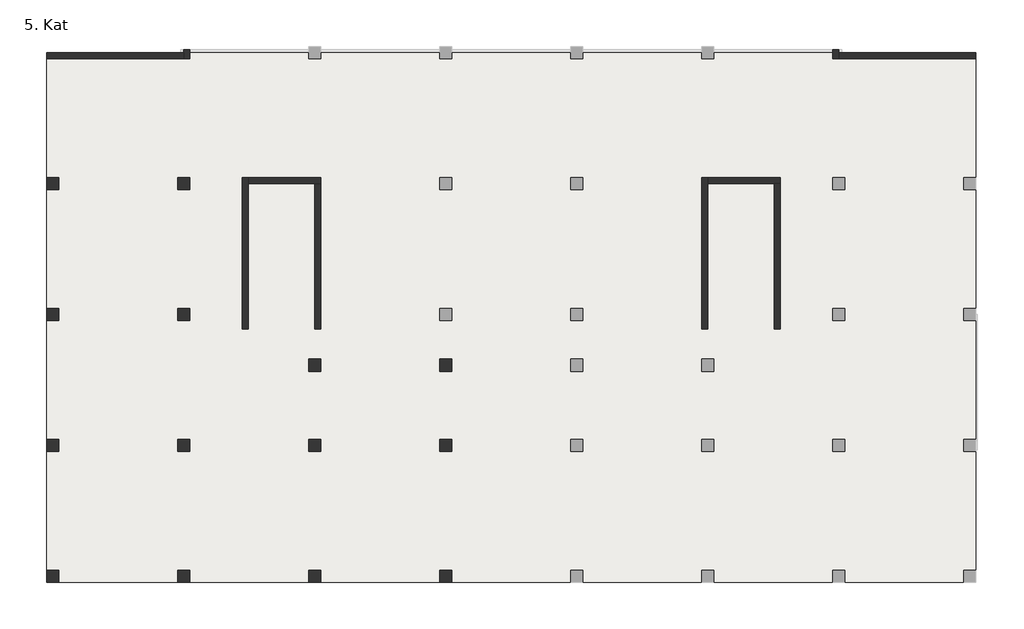
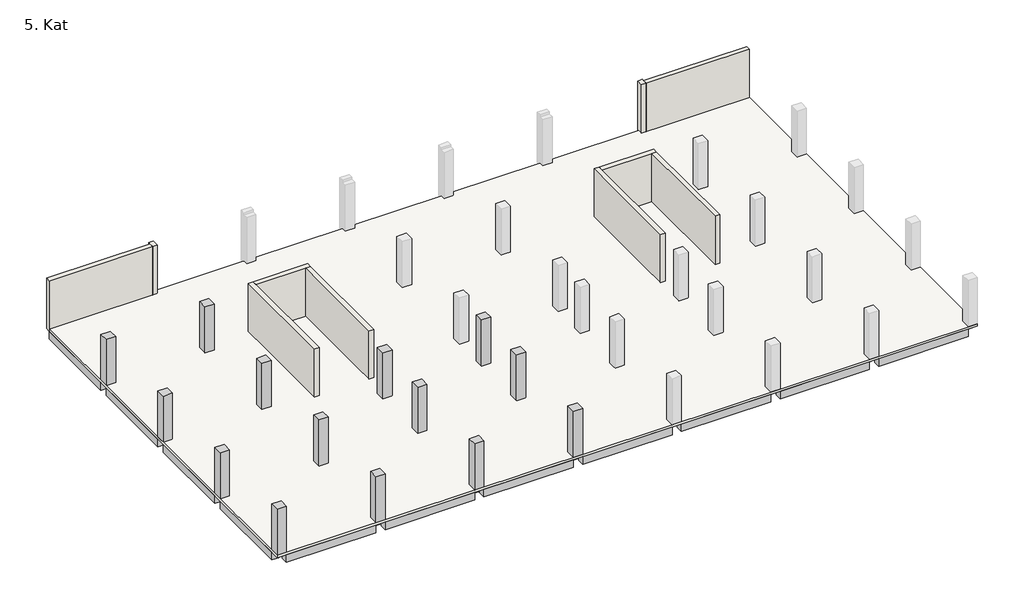
# One storey, part 1 of 2: 41 beams, 14 columns, 10 walls, 1 slab.
"""IFC4 building model written with IfcOpenShell, lengths in millimetres."""

from ifc_helpers import new_model, si_unit, frame, origin, place, context, project, spatial, polyline, outline, extrude, faceted_brep, element, save

model = new_model("IFC4")

# Units and contexts
model_context = context("Model", 3, world=origin())
ifc_project = project(units=[si_unit("LENGTHUNIT", "METRE", prefix="MILLI")], contexts=[model_context])

# Site, building, storey
site = spatial("IfcSite", under=ifc_project)
building = spatial("IfcBuilding", under=site)
storey = spatial("IfcBuildingStorey", under=building, Name="5. Kat", Elevation=26500.0)

# Beams
placement = place(None, origin())
element("IfcBeam", 1, ObjectType="M_Concrete-Rectangular Beam : 60x70cm kiriş", at=placement, inside=storey, context=model_context, shape_type="SweptSolid", body=[
    extrude(outline(polyline([(-400.0003889, 8099.9999582), (199.9996111, 8099.9999582), (199.9996111, 399.9999408), (-400.0003889, 399.9999408), (-400.0003889, 8099.9999582)])), frame((0.0, 0.0, 25800.0), z_axis=(0.0, 0.0, 1.0), x_axis=(1.0, 0.0, 0.0)), (0.0, 0.0, 1.0), 700.0),
])
element("IfcBeam", 2, ObjectType="M_Concrete-Rectangular Beam : 60x70cm kiriş", at=placement, inside=storey, context=model_context, shape_type="SweptSolid", body=[
    extrude(outline(polyline([(-400.0003589, 16599.9999423), (199.9996411, 16599.9999423), (199.9996411, 8899.9999251), (-400.0003589, 8899.9999251), (-400.0003589, 16599.9999423)])), frame((0.0, 0.0, 25800.0), z_axis=(0.0, 0.0, 1.0), x_axis=(1.0, 0.0, 0.0)), (0.0, 0.0, 1.0), 700.0),
])
element("IfcBeam", 3, ObjectType="M_Concrete-Rectangular Beam : 60x70cm kiriş", at=placement, inside=storey, context=model_context, shape_type="Brep", body=[
    faceted_brep([(199.9994072, 25099.999926, 26500.0), (-400.0005928, 25099.999926, 26500.0), (-400.0005928, 17399.9999423, 26500.0), (199.9994072, 17399.9999423, 26500.0), (199.9994072, 23399.9999249, 26500.0), (199.9994072, 23899.9999249, 26500.0), (199.9994072, 25099.999926, 25800.0), (199.9994072, 17399.9999423, 25800.0), (199.9994072, 23399.9999249, 25800.0), (199.9994072, 23899.9999249, 25800.0), (-400.0005928, 25099.999926, 25800.0), (-400.0005928, 17399.9999423, 25800.0)], [[[0, 1, 2, 3, 4, 5]], [[6, 0, 5, 4, 3, 7, 8, 9]], [[10, 6, 9, 8, 7, 11]], [[1, 10, 11, 2]], [[2, 11, 7, 3]], [[1, 0, 6, 10]]]),
])
element("IfcBeam", 4, ObjectType="M_Concrete-Rectangular Beam : 60x70cm kiriş", at=placement, inside=storey, context=model_context, shape_type="SweptSolid", body=[
    extrude(outline(polyline([(199.9994681, 25899.9999188), (-400.0005319, 25899.9999188), (-400.0005319, 33600.0004302), (199.9994681, 33600.0004302), (199.9994681, 25899.9999188)])), frame((0.0, 0.0, 25800.0), z_axis=(0.0, 0.0, 1.0), x_axis=(1.0, 0.0, 0.0)), (0.0, 0.0, 1.0), 700.0),
])
element("IfcBeam", 5, ObjectType="M_Concrete-Rectangular Beam : 60x70cm kiriş", at=placement, inside=storey, context=model_context, shape_type="SweptSolid", body=[
    extrude(outline(polyline([(8099.9996095, 199.9995192), (8099.9996095, -400.0004808), (399.9996111, -400.0004808), (399.9996111, 199.9995192), (8099.9996095, 199.9995192)])), frame((0.0, 0.0, 25800.0), z_axis=(0.0, 0.0, 1.0), x_axis=(1.0, 0.0, 0.0)), (0.0, 0.0, 1.0), 700.0),
])
element("IfcBeam", 6, ObjectType="M_Concrete-Rectangular Beam : 60x70cm kiriş", at=placement, inside=storey, context=model_context, shape_type="SweptSolid", body=[
    extrude(outline(polyline([(16599.9996095, 199.9999577), (16599.9996095, -400.0000423), (8899.9996095, -400.0000423), (8899.9996095, 199.9999577), (16599.9996095, 199.9999577)])), frame((0.0, 0.0, 25800.0), z_axis=(0.0, 0.0, 1.0), x_axis=(1.0, 0.0, 0.0)), (0.0, 0.0, 1.0), 700.0),
])
element("IfcBeam", 7, ObjectType="M_Concrete-Rectangular Beam : 60x70cm kiriş", at=placement, inside=storey, context=model_context, shape_type="SweptSolid", body=[
    extrude(outline(polyline([(25099.9996096, 200.0003837), (25099.9996096, -399.9996163), (17399.9993907, -399.9996163), (17399.9993907, 200.0003837), (25099.9996096, 200.0003837)])), frame((0.0, 0.0, 25800.0), z_axis=(0.0, 0.0, 1.0), x_axis=(1.0, 0.0, 0.0)), (0.0, 0.0, 1.0), 700.0),
])
element("IfcBeam", 8, ObjectType="M_Concrete-Rectangular Beam : 60x70cm kiriş", at=placement, inside=storey, context=model_context, shape_type="SweptSolid", body=[
    extrude(outline(polyline([(8299.9996095, 8100.0003637), (8899.9996095, 8100.0003637), (8899.9996095, 399.9999384), (8299.9996095, 399.9999384), (8299.9996095, 8100.0003637)])), frame((0.0, 0.0, 25800.0), z_axis=(0.0, 0.0, 1.0), x_axis=(1.0, 0.0, 0.0)), (0.0, 0.0, 1.0), 700.0),
])
element("IfcBeam", 9, ObjectType="M_Concrete-Rectangular Beam : 60x70cm kiriş", at=placement, inside=storey, context=model_context, shape_type="Brep", body=[
    faceted_brep([(8899.9996095, 16599.9999418, 26500.0), (8299.9996095, 16599.9999418, 26500.0), (8299.9996095, 8900.0003637, 26500.0), (8899.9996095, 8900.0003637, 26500.0), (8899.9996095, 13300.0003638, 26500.0), (8899.9996095, 13700.0003638, 26500.0), (8899.9996095, 16599.9999418, 25800.0), (8899.9996095, 8900.0003637, 25800.0), (8899.9996095, 13300.0003638, 25800.0), (8899.9996095, 13700.0003638, 25800.0), (8299.9996095, 16599.9999418, 25800.0), (8299.9996095, 8900.0003637, 25800.0)], [[[0, 1, 2, 3, 4, 5]], [[6, 0, 5, 4, 3, 7, 8, 9]], [[10, 6, 9, 8, 7, 11]], [[1, 10, 11, 2]], [[2, 11, 7, 3]], [[1, 0, 6, 10]]]),
])
element("IfcBeam", 10, ObjectType="M_Concrete-Rectangular Beam : 60x70cm kiriş", at=placement, inside=storey, context=model_context, shape_type="Brep", body=[
    faceted_brep([(8899.9996735, 25100.0003646, 26500.0), (8299.9996735, 25100.0003646, 26500.0), (8299.9996735, 23899.9999249, 26500.0), (8299.9996735, 23399.9999249, 26500.0), (8299.9996735, 18550.0006424, 26500.0), (8299.9996735, 18150.0006424, 26500.0), (8299.9996735, 17400.0009197, 26500.0), (8899.9996735, 17400.0009197, 26500.0), (8899.9996735, 25100.0003646, 25800.0), (8899.9996735, 17400.0009197, 25800.0), (8299.9996735, 25100.0003646, 25800.0), (8299.9996735, 17400.0009197, 25800.0), (8299.9996735, 18150.0006424, 25800.0), (8299.9996735, 18550.0006424, 25800.0), (8299.9996735, 23399.9999249, 25800.0), (8299.9996735, 23899.9999249, 25800.0)], [[[0, 1, 2, 3, 4, 5, 6, 7]], [[8, 0, 7, 9]], [[10, 8, 9, 11, 12, 13, 14, 15]], [[1, 10, 15, 14, 13, 12, 11, 6, 5, 4, 3, 2]], [[1, 0, 8, 10]], [[7, 6, 11, 9]]]),
])
element("IfcBeam", 11, ObjectType="M_Concrete-Rectangular Beam : 60x70cm kiriş", at=placement, inside=storey, context=model_context, shape_type="Brep", body=[
    faceted_brep([(8299.9993907, 25899.9999188, 26500.0), (8899.9993907, 25899.9999188, 26500.0), (8899.9993907, 33600.0004302, 26500.0), (8499.9995273, 33600.0004302, 26500.0), (8299.9993907, 33600.0004302, 26500.0), (8899.9993907, 25899.9999188, 25800.0), (8899.9993907, 33600.0004302, 25800.0), (8299.9993907, 25899.9999188, 25800.0), (8299.9993907, 33600.0004302, 25800.0)], [[[0, 1, 2, 3, 4]], [[1, 5, 6, 2]], [[5, 7, 8, 6]], [[7, 0, 4, 8]], [[5, 1, 0, 7]], [[8, 4, 3, 2, 6]]]),
])
element("IfcBeam", 12, ObjectType="M_Concrete-Rectangular Beam : 60x70cm kiriş", at=placement, inside=storey, context=model_context, shape_type="SweptSolid", body=[
    extrude(outline(polyline([(8099.9997323, 25899.999992), (8099.9997323, 25299.999992), (399.9997323, 25299.999992), (399.9997323, 25899.999992), (8099.9997323, 25899.999992)])), frame((0.0, 0.0, 25800.0), z_axis=(0.0, 0.0, 1.0), x_axis=(1.0, 0.0, 0.0)), (0.0, 0.0, 1.0), 700.0),
])
element("IfcBeam", 13, ObjectType="M_Concrete-Rectangular Beam : 50x70cm kiriş", at=placement, inside=storey, context=model_context, shape_type="SweptSolid", body=[
    extrude(outline(polyline([(199.9994072, 23399.9999249), (199.9994072, 23899.9999249), (8299.9996735, 23899.9999249), (8299.9996735, 23399.9999249), (199.9994072, 23399.9999249)])), frame((0.0, 0.0, 25800.0), z_axis=(0.0, 0.0, 1.0), x_axis=(1.0, 0.0, 0.0)), (0.0, 0.0, 1.0), 700.0),
])
element("IfcBeam", 14, ObjectType="M_Concrete-Rectangular Beam : 60x70cm kiriş", at=placement, inside=storey, context=model_context, shape_type="SweptSolid", body=[
    extrude(outline(polyline([(8099.9997451, 8800.0009197), (8099.9997451, 8200.0009197), (399.9996411, 8200.0009197), (399.9996411, 8800.0009197), (8099.9997451, 8800.0009197)])), frame((0.0, 0.0, 25800.0), z_axis=(0.0, 0.0, 1.0), x_axis=(1.0, 0.0, 0.0)), (0.0, 0.0, 1.0), 700.0),
])
element("IfcBeam", 15, ObjectType="M_Concrete-Rectangular Beam : 60x70cm kiriş", at=placement, inside=storey, context=model_context, shape_type="SweptSolid", body=[
    extrude(outline(polyline([(8099.9993907, 17400.0003638), (8099.9993907, 16800.0003638), (400.0000836, 16800.0003638), (400.0000836, 17400.0003638), (8099.9993907, 17400.0003638)])), frame((0.0, 0.0, 25800.0), z_axis=(0.0, 0.0, 1.0), x_axis=(1.0, 0.0, 0.0)), (0.0, 0.0, 1.0), 700.0),
])
element("IfcBeam", 16, ObjectType="M_Concrete-Rectangular Beam : 40x70cm kiriş 2", at=placement, inside=storey, context=model_context, shape_type="SweptSolid", body=[
    extrude(outline(polyline([(204.0222331, 18150.0006424), (204.0222331, 18550.0006424), (8299.9996735, 18550.0006424), (8299.9996735, 18150.0006424), (204.0222331, 18150.0006424)])), frame((0.0, 0.0, 25800.0), z_axis=(0.0, 0.0, 1.0), x_axis=(1.0, 0.0, 0.0)), (0.0, 0.0, 1.0), 700.0),
])
element("IfcBeam", 17, ObjectType="M_Concrete-Rectangular Beam : 60x70cm kiriş", at=placement, inside=storey, context=model_context, shape_type="Brep", body=[
    faceted_brep([(8899.9993907, 25899.9999925, 26500.0), (8899.9993907, 25299.9999925, 26500.0), (12300.0064017, 25299.9999925, 26500.0), (12300.0064017, 25500.0003816, 26500.0), (12300.0064017, 25899.9999925, 26500.0), (8899.9993907, 25299.9999925, 25800.0), (12300.0064017, 25299.9999925, 25800.0), (8899.9993907, 25899.9999925, 25800.0), (12300.0064017, 25899.9999925, 25800.0)], [[[0, 1, 2, 3, 4]], [[1, 5, 6, 2]], [[5, 7, 8, 6]], [[7, 0, 4, 8]], [[0, 7, 5, 1]], [[4, 3, 2, 6, 8]]]),
])
element("IfcBeam", 18, ObjectType="M_Concrete-Rectangular Beam : 60x70cm kiriş", at=placement, inside=storey, context=model_context, shape_type="Brep", body=[
    faceted_brep([(8899.9996735, 17400.0003643, 26500.0), (8899.9993907, 16800.0003643, 26500.0), (12300.0064017, 16800.0003643, 26500.0), (12300.0064017, 17400.0003643, 26500.0), (8899.9993907, 16800.0003643, 25800.0), (12300.0064017, 16800.0003643, 25800.0), (8899.9996735, 17400.0003643, 25800.0), (12300.0064017, 17400.0003643, 25800.0)], [[[0, 1, 2, 3]], [[1, 4, 5, 2]], [[4, 6, 7, 5]], [[6, 0, 3, 7]], [[0, 6, 4, 1]], [[3, 2, 5, 7]]]),
])
element("IfcBeam", 19, ObjectType="M_Concrete-Rectangular Beam : 40x70cm kiriş 2", at=placement, inside=storey, context=model_context, shape_type="Brep", body=[
    faceted_brep([(12700.0064017, 17400.0003638, 26500.0), (12700.0064017, 17000.0003638, 26500.0), (14600.0010318, 17000.0003638, 26500.0), (14900.0010318, 17000.0003638, 26500.0), (16999.9995362, 17000.0003638, 26500.0), (16999.9995362, 17400.0003638, 26500.0), (12700.0064017, 17000.0003638, 25800.0), (14600.0010318, 17000.0003638, 25800.0), (14900.0010318, 17000.0003638, 25800.0), (16999.9995362, 17000.0003638, 25800.0), (12700.0064017, 17400.0003638, 25800.0), (16999.9995362, 17400.0003638, 25800.0)], [[[0, 1, 2, 3, 4, 5]], [[1, 6, 7, 8, 9, 4, 3, 2]], [[6, 10, 11, 9, 8, 7]], [[10, 0, 5, 11]], [[1, 0, 10, 6]], [[5, 4, 9, 11]]]),
])
element("IfcBeam", 20, ObjectType="M_Concrete-Rectangular Beam : 40x70cm kiriş 2", at=placement, inside=storey, context=model_context, shape_type="Brep", body=[
    faceted_brep([(16599.9993867, 13300.0003638, 26500.0), (16599.9993867, 13700.0003638, 26500.0), (14900.0010318, 13700.0003638, 26500.0), (14600.0010318, 13700.0003638, 26500.0), (12700.0064017, 13700.0003638, 26500.0), (12300.0064017, 13700.0003638, 26500.0), (8899.9996095, 13700.0003638, 26500.0), (8899.9996095, 13300.0003638, 26500.0), (12300.0064017, 13300.0003638, 26500.0), (12700.0064017, 13300.0003638, 26500.0), (16599.9993867, 13700.0003638, 25800.0), (14900.0010318, 13700.0003638, 25800.0), (14600.0010318, 13700.0003638, 25800.0), (12700.0064017, 13700.0003638, 25800.0), (12300.0064017, 13700.0003638, 25800.0), (8899.9996095, 13700.0003638, 25800.0), (16599.9993867, 13300.0003638, 25800.0), (12700.0064017, 13300.0003638, 25800.0), (12300.0064017, 13300.0003638, 25800.0), (8899.9996095, 13300.0003638, 25800.0)], [[[0, 1, 2, 3, 4, 5, 6, 7, 8, 9]], [[1, 10, 11, 12, 13, 14, 15, 6, 5, 4, 3, 2]], [[10, 16, 17, 18, 19, 15, 14, 13, 12, 11]], [[16, 0, 9, 8, 7, 19, 18, 17]], [[7, 6, 15, 19]], [[0, 16, 10, 1]]]),
])
element("IfcBeam", 21, ObjectType="M_Concrete-Rectangular Beam : 40x70cm kiriş 2", at=placement, inside=storey, context=model_context, shape_type="SweptSolid", body=[
    extrude(outline(polyline([(12300.0064017, 16037.3003638), (12700.0064017, 16037.3003638), (12700.0064017, 13700.0003638), (12300.0064017, 13700.0003638), (12300.0064017, 16037.3003638)])), frame((0.0, 0.0, 25800.0), z_axis=(0.0, 0.0, 1.0), x_axis=(1.0, 0.0, 0.0)), (0.0, 0.0, 1.0), 700.0),
])
element("IfcBeam", 22, ObjectType="M_Concrete-Rectangular Beam : 40x70cm kiriş 2", at=placement, inside=storey, context=model_context, shape_type="SweptSolid", body=[
    extrude(outline(polyline([(17399.9995362, 14099.9451047), (16999.9995362, 14099.9451047), (16999.9995362, 16037.3003638), (17399.9995362, 16037.3003638), (17399.9995362, 14099.9451047)])), frame((0.0, 0.0, 25800.0), z_axis=(0.0, 0.0, 1.0), x_axis=(1.0, 0.0, 0.0)), (0.0, 0.0, 1.0), 700.0),
])
element("IfcBeam", 23, ObjectType="M_Concrete-Rectangular Beam : 30x70cm kiriş 3", at=placement, inside=storey, context=model_context, shape_type="Brep", body=[
    faceted_brep([(12700.0064017, 16350.0003638, 26500.0), (12700.0064017, 16050.0003638, 26500.0), (14600.0010318, 16050.0003638, 26500.0), (14900.0010318, 16050.0003638, 26500.0), (16999.9995362, 16050.0003638, 26500.0), (16999.9995362, 16350.0003638, 26500.0), (14900.0010318, 16350.0003638, 26500.0), (14600.0010318, 16350.0003638, 26500.0), (12700.0064017, 16350.0003638, 25800.0), (16999.9995362, 16350.0003638, 25800.0), (14900.0010318, 16350.0003638, 25800.0), (14600.0010318, 16350.0003638, 25800.0), (12700.0064017, 16050.0003638, 25800.0), (16999.9995362, 16050.0003638, 25800.0), (14900.0010318, 16050.0003638, 25800.0), (14600.0010318, 16050.0003638, 25800.0)], [[[0, 1, 2, 3, 4, 5, 6, 7]], [[8, 0, 7, 6, 5, 9, 10, 11]], [[12, 8, 11, 10, 9, 13, 14, 15]], [[1, 12, 15, 14, 13, 4, 3, 2]], [[0, 8, 12, 1]], [[5, 4, 13, 9]]]),
])
element("IfcBeam", 24, ObjectType="M_Concrete-Rectangular Beam : 30x70cm kiriş 3", at=placement, inside=storey, context=model_context, shape_type="SweptSolid", body=[
    extrude(outline(polyline([(14900.0010318, 13700.0003638), (14600.0010318, 13700.0003638), (14600.0010318, 16050.0003638), (14900.0010318, 16050.0003638), (14900.0010318, 13700.0003638)])), frame((0.0, 0.0, 25800.0), z_axis=(0.0, 0.0, 1.0), x_axis=(1.0, 0.0, 0.0)), (0.0, 0.0, 1.0), 700.0),
    extrude(outline(polyline([(14600.0010318, 17000.0003638), (14900.0010318, 17000.0003638), (14900.0010318, 16350.0003638), (14600.0010318, 16350.0003638), (14600.0010318, 17000.0003638)])), frame((0.0, 0.0, 25800.0), z_axis=(0.0, 0.0, 1.0), x_axis=(1.0, 0.0, 0.0)), (0.0, 0.0, 1.0), 700.0),
])
element("IfcBeam", 25, ObjectType="M_Concrete-Rectangular Beam : 60x70cm kiriş", at=placement, inside=storey, context=model_context, shape_type="Brep", body=[
    faceted_brep([(16599.9993907, 8200.0009197, 26500.0), (16599.9993907, 8800.0009197, 26500.0), (12700.0064017, 8800.0009197, 26500.0), (12300.0064017, 8800.0009197, 26500.0), (8899.9993907, 8800.0009197, 26500.0), (8899.9993907, 8200.0009197, 26500.0), (16599.9993907, 8200.0009197, 25800.0), (8899.9993907, 8200.0009197, 25800.0), (16599.9993907, 8800.0009197, 25800.0), (8899.9993907, 8800.0009197, 25800.0), (12300.0064017, 8800.0009197, 25800.0), (12700.0064017, 8800.0009197, 25800.0)], [[[0, 1, 2, 3, 4, 5]], [[6, 0, 5, 7]], [[8, 6, 7, 9, 10, 11]], [[1, 8, 11, 10, 9, 4, 3, 2]], [[4, 9, 7, 5]], [[1, 0, 6, 8]]]),
])
element("IfcBeam", 26, ObjectType="M_Concrete-Rectangular Beam : 60x70cm kiriş", at=placement, inside=storey, context=model_context, shape_type="SweptSolid", body=[
    extrude(outline(polyline([(17399.9997293, 8900.0009197), (16799.9997293, 8900.0009197), (16799.9997293, 13299.9451047), (17399.9997293, 13299.9451047), (17399.9997293, 8900.0009197)])), frame((0.0, 0.0, 25800.0), z_axis=(0.0, 0.0, 1.0), x_axis=(1.0, 0.0, 0.0)), (0.0, 0.0, 1.0), 700.0),
])
element("IfcBeam", 27, ObjectType="M_Concrete-Rectangular Beam : 60x70cm kiriş", at=placement, inside=storey, context=model_context, shape_type="SweptSolid", body=[
    extrude(outline(polyline([(17399.9997451, 400.0009197), (16799.9997451, 400.0009197), (16799.9997451, 8099.9999409), (17399.9997451, 8099.9999409), (17399.9997451, 400.0009197)])), frame((0.0, 0.0, 25800.0), z_axis=(0.0, 0.0, 1.0), x_axis=(1.0, 0.0, 0.0)), (0.0, 0.0, 1.0), 700.0),
])
element("IfcBeam", 28, ObjectType="M_Concrete-Rectangular Beam : 40x70cm kiriş 2", at=placement, inside=storey, context=model_context, shape_type="SweptSolid", body=[
    extrude(outline(polyline([(12300.0064017, 13300.0003638), (12700.0064017, 13300.0003638), (12700.0064017, 8800.0009197), (12300.0064017, 8800.0009197), (12300.0064017, 13300.0003638)])), frame((0.0, 0.0, 25800.0), z_axis=(0.0, 0.0, 1.0), x_axis=(1.0, 0.0, 0.0)), (0.0, 0.0, 1.0), 700.0),
])
element("IfcBeam", 29, ObjectType="M_Concrete-Rectangular Beam : 60x70cm kiriş", at=placement, inside=storey, context=model_context, shape_type="SweptSolid", body=[
    extrude(outline(polyline([(25899.9997233, 400.0009197), (25299.9997233, 400.0009197), (25299.9997233, 8100.0009197), (25899.9997233, 8100.0009197), (25899.9997233, 400.0009197)])), frame((0.0, 0.0, 25800.0), z_axis=(0.0, 0.0, 1.0), x_axis=(1.0, 0.0, 0.0)), (0.0, 0.0, 1.0), 700.0),
])
element("IfcBeam", 30, ObjectType="M_Concrete-Rectangular Beam : 60x70cm kiriş", at=placement, inside=storey, context=model_context, shape_type="SweptSolid", body=[
    extrude(outline(polyline([(25099.9993907, 8800.0009197), (25099.9993907, 8200.0009197), (17399.9993907, 8200.0009197), (17399.9993907, 8800.0009197), (25099.9993907, 8800.0009197)])), frame((0.0, 0.0, 25800.0), z_axis=(0.0, 0.0, 1.0), x_axis=(1.0, 0.0, 0.0)), (0.0, 0.0, 1.0), 700.0),
])
element("IfcBeam", 31, ObjectType="M_Concrete-Rectangular Beam : 60x70cm kiriş", at=placement, inside=storey, context=model_context, shape_type="SweptSolid", body=[
    extrude(outline(polyline([(25899.9997233, 8900.0009197), (25299.9997233, 8900.0009197), (25299.9997233, 13300.0003995), (25899.9997233, 13300.0003995), (25899.9997233, 8900.0009197)])), frame((0.0, 0.0, 25800.0), z_axis=(0.0, 0.0, 1.0), x_axis=(1.0, 0.0, 0.0)), (0.0, 0.0, 1.0), 700.0),
])
element("IfcBeam", 32, ObjectType="M_Concrete-Rectangular Beam : 40x70cm kiriş 2", at=placement, inside=storey, context=model_context, shape_type="Brep", body=[
    faceted_brep([(17399.9993907, 13700.0003995, 26500.0), (17399.9997293, 13300.0003995, 26500.0), (25099.9997415, 13300.0003995, 26500.0), (25099.9997415, 13700.0003995, 26500.0), (25099.9997415, 13700.0003995, 25800.0), (17399.9993907, 13700.0003995, 25800.0), (17399.9997293, 13300.0003995, 25800.0), (25099.9997415, 13300.0003995, 25800.0)], [[[0, 1, 2, 3]], [[3, 4, 5, 0]], [[6, 5, 4, 7]], [[1, 6, 7, 2]], [[0, 5, 6, 1]], [[2, 7, 4, 3]]]),
])
element("IfcBeam", 33, ObjectType="M_Concrete-Rectangular Beam : 60x70cm kiriş", at=placement, inside=storey, context=model_context, shape_type="SweptSolid", body=[
    extrude(outline(polyline([(25899.9997233, 14100.0003995), (25299.9997233, 14100.0003995), (25299.9997233, 16600.0009197), (25899.9997233, 16600.0009197), (25899.9997233, 14100.0003995)])), frame((0.0, 0.0, 25800.0), z_axis=(0.0, 0.0, 1.0), x_axis=(1.0, 0.0, 0.0)), (0.0, 0.0, 1.0), 700.0),
])
element("IfcBeam", 34, ObjectType="M_Concrete-Rectangular Beam : 40x70cm kiriş 2", at=placement, inside=storey, context=model_context, shape_type="Brep", body=[
    faceted_brep([(25899.9993907, 13700.0003995, 26500.0), (25899.9997233, 13300.0003995, 26500.0), (33599.9993907, 13300.0003995, 26500.0), (33599.9993907, 13700.0003995, 26500.0), (25899.9997233, 13300.0003995, 25800.0), (33599.9993907, 13300.0003995, 25800.0), (25899.9993907, 13700.0003995, 25800.0), (33599.9993907, 13700.0003995, 25800.0)], [[[0, 1, 2, 3]], [[1, 4, 5, 2]], [[4, 6, 7, 5]], [[3, 7, 6, 0]], [[0, 6, 4, 1]], [[2, 5, 7, 3]]]),
])
element("IfcBeam", 35, ObjectType="M_Concrete-Rectangular Beam : 60x70cm kiriş", at=placement, inside=storey, context=model_context, shape_type="Brep", body=[
    faceted_brep([(33599.9993907, 8200.0009197, 26500.0), (33599.9994953, 8800.0009197, 26500.0), (25899.9993907, 8800.0009197, 26500.0), (25899.9993907, 8200.0009197, 26500.0), (25899.9993907, 8200.0009197, 25800.0), (33599.9993907, 8200.0009197, 25800.0), (33599.9994953, 8800.0009197, 25800.0), (25899.9993907, 8800.0009197, 25800.0)], [[[0, 1, 2, 3]], [[3, 4, 5, 0]], [[6, 5, 4, 7]], [[1, 6, 7, 2]], [[0, 5, 6, 1]], [[4, 3, 2, 7]]]),
])
element("IfcBeam", 36, ObjectType="M_Concrete-Rectangular Beam : 60x70cm kiriş", at=placement, inside=storey, context=model_context, shape_type="Brep", body=[
    faceted_brep([(42099.9993899, -399.9996882, 26500.0), (42099.999723, 200.0003118, 26500.0), (34399.9993907, 200.0003118, 26500.0), (34399.9993907, -399.9996882, 26500.0), (34399.9993907, -399.9996882, 25800.0), (42099.9993899, -399.9996882, 25800.0), (42099.999723, 200.0003118, 25800.0), (34399.9993907, 200.0003118, 25800.0)], [[[0, 1, 2, 3]], [[3, 4, 5, 0]], [[6, 5, 4, 7]], [[1, 6, 7, 2]], [[0, 5, 6, 1]], [[4, 3, 2, 7]]]),
])
element("IfcBeam", 37, ObjectType="M_Concrete-Rectangular Beam : 60x70cm kiriş", at=placement, inside=storey, context=model_context, shape_type="SweptSolid", body=[
    extrude(outline(polyline([(25899.9993907, -399.9996882), (25899.9993907, 200.0003118), (33599.9993907, 200.0003118), (33599.9993907, -399.9996882), (25899.9993907, -399.9996882)])), frame((0.0, 0.0, 25800.0), z_axis=(0.0, 0.0, 1.0), x_axis=(1.0, 0.0, 0.0)), (0.0, 0.0, 1.0), 700.0),
])
element("IfcBeam", 38, ObjectType="M_Concrete-Rectangular Beam : 60x70cm kiriş", at=placement, inside=storey, context=model_context, shape_type="Brep", body=[
    faceted_brep([(50599.9993899, -399.9996882, 26500.0), (50599.999723, 200.0003118, 26500.0), (42899.9997771, 200.0003118, 26500.0), (42899.9997771, -399.9996882, 26500.0), (42899.9997771, -399.9996882, 25800.0), (50599.9993899, -399.9996882, 25800.0), (50599.999723, 200.0003118, 25800.0), (42899.9997771, 200.0003118, 25800.0)], [[[0, 1, 2, 3]], [[3, 4, 5, 0]], [[6, 5, 4, 7]], [[1, 6, 7, 2]], [[0, 5, 6, 1]], [[2, 7, 4, 3]]]),
])
element("IfcBeam", 39, ObjectType="M_Concrete-Rectangular Beam : 60x70cm kiriş", at=placement, inside=storey, context=model_context, shape_type="SweptSolid", body=[
    extrude(outline(polyline([(59099.9997769, 200.0003118), (59099.9997769, -399.9996882), (51399.9997769, -399.9996882), (51399.9997769, 200.0003118), (59099.9997769, 200.0003118)])), frame((0.0, 0.0, 25800.0), z_axis=(0.0, 0.0, 1.0), x_axis=(1.0, 0.0, 0.0)), (0.0, 0.0, 1.0), 700.0),
])
element("IfcBeam", 40, ObjectType="M_Concrete-Rectangular Beam : 40x70cm kiriş 2", at=placement, inside=storey, context=model_context, shape_type="SweptSolid", body=[
    extrude(outline(polyline([(12300.0064017, 16050.000156), (12700.0064017, 16050.000156), (12700.0064017, 16037.3003638), (12300.0064017, 16037.3003638), (12300.0064017, 16050.000156)])), frame((0.0, 0.0, 25800.0), z_axis=(0.0, 0.0, 1.0), x_axis=(1.0, 0.0, 0.0)), (0.0, 0.0, 1.0), 700.0),
])
element("IfcBeam", 41, ObjectType="M_Concrete-Rectangular Beam : 40x70cm kiriş 2", at=placement, inside=storey, context=model_context, shape_type="SweptSolid", body=[
    extrude(outline(polyline([(16999.9995362, 16050.0003816), (17399.9995362, 16050.0003816), (17399.9995362, 16037.3003638), (16999.9995362, 16037.3003638), (16999.9995362, 16050.0003816)])), frame((0.0, 0.0, 25800.0), z_axis=(0.0, 0.0, 1.0), x_axis=(1.0, 0.0, 0.0)), (0.0, 0.0, 1.0), 700.0),
])

# Columns
element("IfcColumn", 42, ObjectType="M_Concrete-Rectangular-Column : 80x80cm kolon", at=placement, inside=storey, context=model_context, shape_type="SweptSolid", body=[
    extrude(outline(polyline([(400.0000836, 400.0009197), (400.0000836, -399.9990803), (-399.9999164, -399.9990803), (-399.9999164, 400.0009197), (400.0000836, 400.0009197)])), frame((0.0, 0.0, 26700.0), z_axis=(0.0, 0.0, 1.0), x_axis=(1.0, 0.0, 0.0)), (0.0, 0.0, 1.0), 4200.0),
])
element("IfcColumn", 43, ObjectType="M_Concrete-Rectangular-Column : 80x80cm kolon", at=placement, inside=storey, context=model_context, shape_type="SweptSolid", body=[
    extrude(outline(polyline([(8899.9993907, 400.0009197), (8899.9993907, -399.9990803), (8099.9993907, -399.9990803), (8099.9993907, 400.0009197), (8899.9993907, 400.0009197)])), frame((0.0, 0.0, 26700.0), z_axis=(0.0, 0.0, 1.0), x_axis=(1.0, 0.0, 0.0)), (0.0, 0.0, 1.0), 4200.0),
])
element("IfcColumn", 44, ObjectType="M_Concrete-Rectangular-Column : 80x80cm kolon", at=placement, inside=storey, context=model_context, shape_type="SweptSolid", body=[
    extrude(outline(polyline([(400.0000836, 8900.0009197), (400.0000836, 8100.0009197), (-399.9999164, 8100.0009197), (-399.9999164, 8900.0009197), (400.0000836, 8900.0009197)])), frame((0.0, 0.0, 26700.0), z_axis=(0.0, 0.0, 1.0), x_axis=(1.0, 0.0, 0.0)), (0.0, 0.0, 1.0), 4200.0),
])
element("IfcColumn", 45, ObjectType="M_Concrete-Rectangular-Column : 80x80cm kolon", at=placement, inside=storey, context=model_context, shape_type="SweptSolid", body=[
    extrude(outline(polyline([(8899.9993907, 8900.0009197), (8899.9993907, 8100.0009197), (8099.9993907, 8100.0009197), (8099.9993907, 8900.0009197), (8899.9993907, 8900.0009197)])), frame((0.0, 0.0, 26700.0), z_axis=(0.0, 0.0, 1.0), x_axis=(1.0, 0.0, 0.0)), (0.0, 0.0, 1.0), 4200.0),
])
element("IfcColumn", 46, ObjectType="M_Concrete-Rectangular-Column : 80x80cm kolon", at=placement, inside=storey, context=model_context, shape_type="SweptSolid", body=[
    extrude(outline(polyline([(8899.9993907, 17400.0009197), (8899.9993907, 16600.0009197), (8099.9993907, 16600.0009197), (8099.9993907, 17400.0009197), (8899.9993907, 17400.0009197)])), frame((0.0, 0.0, 26700.0), z_axis=(0.0, 0.0, 1.0), x_axis=(1.0, 0.0, 0.0)), (0.0, 0.0, 1.0), 4200.0),
])
element("IfcColumn", 47, ObjectType="M_Concrete-Rectangular-Column : 80x80cm kolon", at=placement, inside=storey, context=model_context, shape_type="SweptSolid", body=[
    extrude(outline(polyline([(400.0000836, 17400.0009197), (400.0000836, 16600.0009197), (-399.9999164, 16600.0009197), (-399.9999164, 17400.0009197), (400.0000836, 17400.0009197)])), frame((0.0, 0.0, 26700.0), z_axis=(0.0, 0.0, 1.0), x_axis=(1.0, 0.0, 0.0)), (0.0, 0.0, 1.0), 4200.0),
])
element("IfcColumn", 48, ObjectType="M_Concrete-Rectangular-Column : 80x80cm kolon", at=placement, inside=storey, context=model_context, shape_type="SweptSolid", body=[
    extrude(outline(polyline([(399.9996699, 25899.9999188), (399.9996699, 25099.9999188), (-400.0003301, 25099.9999188), (-400.0003301, 25899.9999188), (399.9996699, 25899.9999188)])), frame((0.0, 0.0, 26700.0), z_axis=(0.0, 0.0, 1.0), x_axis=(1.0, 0.0, 0.0)), (0.0, 0.0, 1.0), 4200.0),
])
element("IfcColumn", 49, ObjectType="M_Concrete-Rectangular-Column : 80x80cm kolon", at=placement, inside=storey, context=model_context, shape_type="SweptSolid", body=[
    extrude(outline(polyline([(8899.9993907, 25899.9999188), (8899.9993907, 25099.9999188), (8099.9993907, 25099.9999188), (8099.9993907, 25899.9999188), (8899.9993907, 25899.9999188)])), frame((0.0, 0.0, 26700.0), z_axis=(0.0, 0.0, 1.0), x_axis=(1.0, 0.0, 0.0)), (0.0, 0.0, 1.0), 4200.0),
])
element("IfcColumn", 50, ObjectType="M_Concrete-Rectangular-Column : 80x80cm kolon", at=placement, inside=storey, context=model_context, shape_type="SweptSolid", body=[
    extrude(outline(polyline([(17399.9993907, 8900.0009197), (17399.9993907, 8100.0009197), (16599.9993907, 8100.0009197), (16599.9993907, 8900.0009197), (17399.9993907, 8900.0009197)])), frame((0.0, 0.0, 26700.0), z_axis=(0.0, 0.0, 1.0), x_axis=(1.0, 0.0, 0.0)), (0.0, 0.0, 1.0), 4200.0),
])
element("IfcColumn", 51, ObjectType="M_Concrete-Rectangular-Column : 80x80cm kolon", at=placement, inside=storey, context=model_context, shape_type="SweptSolid", body=[
    extrude(outline(polyline([(25899.9993907, 8900.0009197), (25899.9993907, 8100.0009197), (25099.9993907, 8100.0009197), (25099.9993907, 8900.0009197), (25899.9993907, 8900.0009197)])), frame((0.0, 0.0, 26700.0), z_axis=(0.0, 0.0, 1.0), x_axis=(1.0, 0.0, 0.0)), (0.0, 0.0, 1.0), 4200.0),
])
element("IfcColumn", 52, ObjectType="M_Concrete-Rectangular-Column : 80x80cm kolon", at=placement, inside=storey, context=model_context, shape_type="SweptSolid", body=[
    extrude(outline(polyline([(25899.9993907, 400.0009197), (25899.9993907, -399.9990803), (25099.9993907, -399.9990803), (25099.9993907, 400.0009197), (25899.9993907, 400.0009197)])), frame((0.0, 0.0, 26700.0), z_axis=(0.0, 0.0, 1.0), x_axis=(1.0, 0.0, 0.0)), (0.0, 0.0, 1.0), 4200.0),
])
element("IfcColumn", 53, ObjectType="M_Concrete-Rectangular-Column : 80x80cm kolon", at=placement, inside=storey, context=model_context, shape_type="SweptSolid", body=[
    extrude(outline(polyline([(17399.9993907, 400.0009197), (17399.9993907, -399.9990803), (16599.9993907, -399.9990803), (16599.9993907, 400.0009197), (17399.9993907, 400.0009197)])), frame((0.0, 0.0, 26700.0), z_axis=(0.0, 0.0, 1.0), x_axis=(1.0, 0.0, 0.0)), (0.0, 0.0, 1.0), 4200.0),
])
element("IfcColumn", 54, ObjectType="M_Concrete-Rectangular-Column : 80x80cm kolon", at=placement, inside=storey, context=model_context, shape_type="SweptSolid", body=[
    extrude(outline(polyline([(25899.9993907, 14100.0003995), (25899.9993907, 13300.0003995), (25099.9993907, 13300.0003995), (25099.9993907, 14100.0003995), (25899.9993907, 14100.0003995)])), frame((0.0, 0.0, 26700.0), z_axis=(0.0, 0.0, 1.0), x_axis=(1.0, 0.0, 0.0)), (0.0, 0.0, 1.0), 4200.0),
])
element("IfcColumn", 55, ObjectType="M_Concrete-Rectangular-Column : 80x80cm kolon", at=placement, inside=storey, context=model_context, shape_type="SweptSolid", body=[
    extrude(outline(polyline([(17399.9993907, 14099.9451047), (17399.9993907, 13299.9451047), (16599.9993907, 13299.9451047), (16599.9993907, 14099.9451047), (17399.9993907, 14099.9451047)])), frame((0.0, 0.0, 26700.0), z_axis=(0.0, 0.0, 1.0), x_axis=(1.0, 0.0, 0.0)), (0.0, 0.0, 1.0), 4200.0),
])

# Slab
element("IfcSlab", 56, ObjectType="20 cm döşeme", at=placement, inside=storey, context=model_context, shape_type="Brep", body=[
    faceted_brep([(59899.9997758, 34000.0004302, 26500.0), (59899.9997758, -399.9995292, 26500.0), (-400.0005319, -399.9995292, 26500.0), (-400.0005319, 25899.9999188, 26500.0), (-400.0005319, 33600.0004302, 26500.0), (-400.0005319, 34000.0004302, 26500.0), (16599.9993907, 34000.0004302, 26500.0), (17399.9993907, 34000.0004302, 26500.0), (25099.9993907, 34000.0004302, 26500.0), (25899.9993907, 34000.0004302, 26500.0), (33599.9993907, 34000.0004302, 26500.0), (34399.9993907, 34000.0004302, 26500.0), (42099.9993899, 34000.0004302, 26500.0), (42899.9993899, 34000.0004302, 26500.0), (59899.9997758, 34000.0004302, 26700.0), (42899.9993899, 34000.0004302, 26700.0), (42099.9993899, 34000.0004302, 26700.0), (34399.9993907, 34000.0004302, 26700.0), (33599.9993907, 34000.0004302, 26700.0), (25899.9993907, 34000.0004302, 26700.0), (25099.9993907, 34000.0004302, 26700.0), (17399.9993907, 34000.0004302, 26700.0), (16599.9993907, 34000.0004302, 26700.0), (-400.0005319, 34000.0004302, 26700.0), (-400.0005319, -399.9995292, 26700.0), (59899.9997758, -399.9995292, 26700.0)], [[[0, 1, 2, 3, 4, 5, 6, 7, 8, 9, 10, 11, 12, 13]], [[14, 15, 16, 17, 18, 19, 20, 21, 22, 23, 24, 25]], [[1, 0, 14, 25]], [[2, 1, 25, 24]], [[5, 4, 3, 2, 24, 23]], [[0, 13, 12, 11, 10, 9, 8, 7, 6, 5, 23, 22, 21, 20, 19, 18, 17, 16, 15, 14]]]),
])

# Walls
element("IfcWall", 57, ObjectType="40cm perde duvar", at=placement, inside=storey, context=model_context, shape_type="SweptSolid", body=[
    extrude(outline(polyline([(8499.9995273, 33600.0004302), (-400.0005319, 33600.0004302), (-400.0005319, 34000.0004302), (8499.9995273, 34000.0004302), (8499.9995273, 33600.0004302)])), frame((0.0, 0.0, 26500.0), z_axis=(0.0, 0.0, 1.0), x_axis=(1.0, 0.0, 0.0)), (0.0, 0.0, 1.0), 4600.0),
])
element("IfcWall", 58, ObjectType="40cm perde duvar", at=placement, inside=storey, context=model_context, shape_type="Brep", body=[
    faceted_brep([(8899.9995273, 33600.0004302, 26500.0), (8899.9995273, 34200.0004302, 26500.0), (8899.9995273, 34200.0004302, 31100.0), (8899.9995273, 33600.0004302, 31100.0), (8499.9995273, 33600.0004302, 26500.0), (8499.9995273, 33600.0004302, 31100.0), (8499.9995273, 34000.0004302, 31100.0), (8499.9995273, 34200.0004302, 31100.0), (8499.9995273, 34200.0004302, 26500.0), (8499.9995273, 34000.0004302, 26500.0)], [[[0, 1, 2, 3]], [[4, 5, 6, 7, 8, 9]], [[1, 0, 4, 9, 8]], [[2, 1, 8, 7]], [[3, 2, 7, 6, 5]], [[0, 3, 5, 4]]]),
])
element("IfcWall", 59, ObjectType="40cm perde duvar", at=placement, inside=storey, context=model_context, shape_type="Brep", body=[
    faceted_brep([(12700.0064017, 16050.000156, 26500.0), (12700.0064017, 25500.0003816, 26500.0), (12700.0064017, 25900.0003816, 26500.0), (12700.0064017, 25900.0003816, 31100.0), (12700.0064017, 25500.0003816, 31100.0), (12700.0064017, 16050.000156, 31100.0), (12300.0064017, 16050.000156, 26500.0), (12300.0064017, 16050.000156, 31100.0), (12300.0064017, 25900.0003816, 31100.0), (12300.0064017, 25900.0003816, 26500.0)], [[[0, 1, 2, 3, 4, 5]], [[6, 7, 8, 9]], [[2, 1, 0, 6, 9]], [[5, 4, 3, 8, 7]], [[0, 5, 7, 6]], [[3, 2, 9, 8]]]),
])
element("IfcWall", 60, ObjectType="40cm perde duvar", at=placement, inside=storey, context=model_context, shape_type="Brep", body=[
    faceted_brep([(12700.0064017, 25500.0003816, 26500.0), (16999.9995362, 25500.0003816, 26500.0), (17399.9995362, 25500.0003816, 26500.0), (17399.9995362, 25500.0003816, 31100.0), (16999.9995362, 25500.0003816, 31100.0), (12700.0064017, 25500.0003816, 31100.0), (12700.0064017, 25900.0003816, 26500.0), (12700.0064017, 25900.0003816, 31100.0), (17399.9995362, 25900.0003816, 31100.0), (17399.9995362, 25900.0003816, 26500.0)], [[[0, 1, 2, 3, 4, 5]], [[6, 7, 8, 9]], [[2, 1, 0, 6, 9]], [[5, 4, 3, 8, 7]], [[0, 5, 7, 6]], [[3, 2, 9, 8]]]),
])
element("IfcWall", 61, ObjectType="40cm perde duvar", at=placement, inside=storey, context=model_context, shape_type="SweptSolid", body=[
    extrude(outline(polyline([(16999.9995362, 16050.0003816), (16999.9995362, 25500.0003816), (17399.9995362, 25500.0003816), (17399.9995362, 16050.0003816), (16999.9995362, 16050.0003816)])), frame((0.0, 0.0, 26500.0), z_axis=(0.0, 0.0, 1.0), x_axis=(1.0, 0.0, 0.0)), (0.0, 0.0, 1.0), 4600.0),
])
element("IfcWall", 62, ObjectType="40cm perde duvar", at=placement, inside=storey, context=model_context, shape_type="Brep", body=[
    faceted_brep([(42499.9995162, 16050.0004138, 26500.0), (42499.9995162, 25500.0004459, 26500.0), (42499.9995162, 25900.0004459, 26500.0), (42499.9995162, 25900.0004459, 31100.0), (42499.9995162, 25500.0004459, 31100.0), (42499.9995162, 16050.0004138, 31100.0), (42499.9995162, 16050.0004138, 30900.0), (42499.9995162, 16050.0004138, 30400.0), (42099.9995162, 16050.0004138, 26500.0), (42099.9995162, 16050.0004138, 30400.0), (42099.9995162, 16050.0004138, 30900.0), (42099.9995162, 16050.0004138, 31100.0), (42099.9995162, 25900.0004459, 31100.0), (42099.9995162, 25900.0004459, 26500.0)], [[[0, 1, 2, 3, 4, 5, 6, 7]], [[8, 9, 10, 11, 12, 13]], [[2, 1, 0, 8, 13]], [[5, 4, 3, 12, 11]], [[0, 7, 6, 5, 11, 10, 9, 8]], [[3, 2, 13, 12]]]),
])
element("IfcWall", 63, ObjectType="40cm perde duvar", at=placement, inside=storey, context=model_context, shape_type="Brep", body=[
    faceted_brep([(42499.9995162, 25500.0004459, 26500.0), (46799.999381, 25500.0004459, 26500.0), (47199.999381, 25500.0004459, 26500.0), (47199.999381, 25500.0004459, 31100.0), (46799.999381, 25500.0004459, 31100.0), (42499.9995162, 25500.0004459, 31100.0), (42499.9995162, 25900.0004459, 26500.0), (42499.9995162, 25900.0004459, 31100.0), (47199.999381, 25900.0004459, 31100.0), (47199.999381, 25900.0004459, 26500.0)], [[[0, 1, 2, 3, 4, 5]], [[6, 7, 8, 9]], [[2, 1, 0, 6, 9]], [[5, 4, 3, 8, 7]], [[0, 5, 7, 6]], [[3, 2, 9, 8]]]),
])
element("IfcWall", 64, ObjectType="40cm perde duvar", at=placement, inside=storey, context=model_context, shape_type="Brep", body=[
    faceted_brep([(46799.999381, 25500.0004459, 26500.0), (46799.999381, 16050.0004138, 26500.0), (46799.999381, 16050.0004138, 30400.0), (46799.999381, 16050.0004138, 30900.0), (46799.999381, 16050.0004138, 31100.0), (46799.999381, 25500.0004459, 31100.0), (47199.999381, 25500.0004459, 26500.0), (47199.999381, 25500.0004459, 31100.0), (47199.999381, 16050.0004138, 31100.0), (47199.999381, 16050.0004138, 30900.0), (47199.999381, 16050.0004138, 30400.0), (47199.999381, 16050.0004138, 26500.0)], [[[0, 1, 2, 3, 4, 5]], [[6, 7, 8, 9, 10, 11]], [[1, 0, 6, 11]], [[4, 3, 2, 1, 11, 10, 9, 8]], [[5, 4, 8, 7]], [[0, 5, 7, 6]]]),
])
element("IfcWall", 65, ObjectType="40cm perde duvar", at=placement, inside=storey, context=model_context, shape_type="Brep", body=[
    faceted_brep([(50599.9994944, 34193.7257565, 26500.0), (50599.9994944, 33600.0004303, 26500.0), (50599.9994944, 33600.0004303, 31100.0), (50599.9994944, 34193.7257565, 31100.0), (50999.9994944, 34193.7257565, 26500.0), (50999.9994944, 34193.7257565, 31100.0), (50999.9994944, 34000.0004303, 31100.0), (50999.9994944, 33600.0004303, 31100.0), (50999.9994944, 33600.0004303, 26500.0), (50999.9994944, 34000.0004303, 26500.0)], [[[0, 1, 2, 3]], [[4, 5, 6, 7, 8, 9]], [[1, 0, 4, 9, 8]], [[3, 2, 7, 6, 5]], [[0, 3, 5, 4]], [[2, 1, 8, 7]]]),
])
element("IfcWall", 66, ObjectType="40cm perde duvar", at=placement, inside=storey, context=model_context, shape_type="SweptSolid", body=[
    extrude(outline(polyline([(59899.9999497, 33600.0004303), (50999.9994944, 33600.0004303), (50999.9994944, 34000.0004303), (59899.9999497, 34000.0004303), (59899.9999497, 33600.0004303)])), frame((0.0, 0.0, 26500.0), z_axis=(0.0, 0.0, 1.0), x_axis=(1.0, 0.0, 0.0)), (0.0, 0.0, 1.0), 4600.0),
])

save(model, "model.ifc")

# Revit data of these elements
# Type "M_Concrete-Rectangular Beam : 60x70cm kiriş"
#   Length [instance default] = 152.4 cm
#   b = 60 cm
#   h = 70 cm
#   Structural Material [instance default] = Concrete, Cast-in-Place gray
#   Assembly Code = ""
# Type "M_Concrete-Rectangular Beam : 50x70cm kiriş"
#   Length [instance default] = 152.4 cm
#   b = 50 cm
#   h = 70 cm
#   Structural Material [instance default] = Concrete, Cast-in-Place gray
#   Assembly Code = ""
# Type "M_Concrete-Rectangular Beam : 40x70cm kiriş 2"
#   Length [instance default] = 152.4 cm
#   b = 40 cm
#   h = 70 cm
#   Structural Material [instance default] = Concrete, Cast-in-Place gray
#   Assembly Code = ""
# Type "M_Concrete-Rectangular Beam : 30x70cm kiriş 3"
#   Length [instance default] = 152.4 cm
#   b = 30 cm
#   h = 70 cm
#   Structural Material [instance default] = Concrete, Cast-in-Place gray
#   Assembly Code = ""
# Type "M_Concrete-Rectangular-Column : 80x80cm kolon"
#   b = 80 cm
#   h = 80 cm
#   Structural Material [instance default] = Concrete, Cast-in-Place gray
# Type "20 cm döşeme"
#   Function = 0
#   Layers, outside or top first: 20 cm no material (function 1)
# Type "40cm perde duvar"
#   Layers, outside or top first: 40 cm no material (function 1)
# Elements 1, 2, 3, 4, 5, 6, 7, 8, 9, 10, 11, 12, 14, 15, 17, 18, 25, 26, 27, 29, 30, 31, 33, 35, 36, 37, 38, 39 (IfcBeam, "M_Concrete-Rectangular Beam : 60x70cm kiriş")
#   Comments = ""
#   Structural Material = Concrete, Cast-in-Place gray
#   Phase Created = New Construction
#   Materials on its faces: "Concrete, Cast-in-Place gray"
# Element 13 (IfcBeam, "M_Concrete-Rectangular Beam : 50x70cm kiriş")
#   Comments = ""
#   Structural Material = Concrete, Cast-in-Place gray
#   Phase Created = New Construction
#   Materials on its faces: "Concrete, Cast-in-Place gray"
# Elements 16, 19, 20, 21, 22, 28, 32, 34, 40, 41 (IfcBeam, "M_Concrete-Rectangular Beam : 40x70cm kiriş 2")
#   Comments = ""
#   Structural Material = Concrete, Cast-in-Place gray
#   Phase Created = New Construction
#   Materials on its faces: "Concrete, Cast-in-Place gray"
# Elements 23, 24 (IfcBeam, "M_Concrete-Rectangular Beam : 30x70cm kiriş 3")
#   Comments = ""
#   Structural Material = Concrete, Cast-in-Place gray
#   Phase Created = New Construction
#   Materials on its faces: "Concrete, Cast-in-Place gray"
# Elements 42, 43, 44, 45, 46, 47, 48, 49, 50, 51, 52, 53, 54, 55 (IfcColumn, "M_Concrete-Rectangular-Column : 80x80cm kolon")
#   Structural Material = Concrete, Cast-in-Place gray
#   Phase Created = New Construction
#   Materials on its faces: "Concrete, Cast-in-Place gray"
# Element 56 (IfcSlab, "20 cm döşeme")
#   Height Offset From Level = 20 cm
#   built-in parameter 1001954 = 1
#   Phase Created = New Construction
#   Materials on its faces: "Default Floor"
# Elements 57, 58, 59, 60, 61, 62, 63, 64, 65, 66 (IfcWall, "40cm perde duvar")
#   Comments = ""
#   Top Offset = 460 cm
#   Base Offset = 0 cm
#   wall height = 460 cm
#   Phase Created = New Construction
#   Base Constraint = 5. Kat
#   Top Constraint = 5. Kat
#   Materials on its faces: "Default Wall"
# Materials
#   "Concrete, Cast-in-Place gray": class "Concrete", colour RGB 192 192 192, transparency 0, Description = "Cast-in-place concrete", Cost = 0
#   "Default Floor": class "Miscellaneous", colour RGB 127 127 127, transparency 0
#   "Default Wall": class "Miscellaneous", colour RGB 128 128 128, transparency 0
